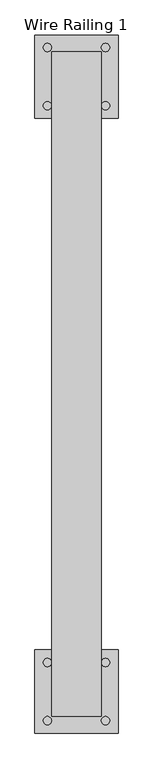
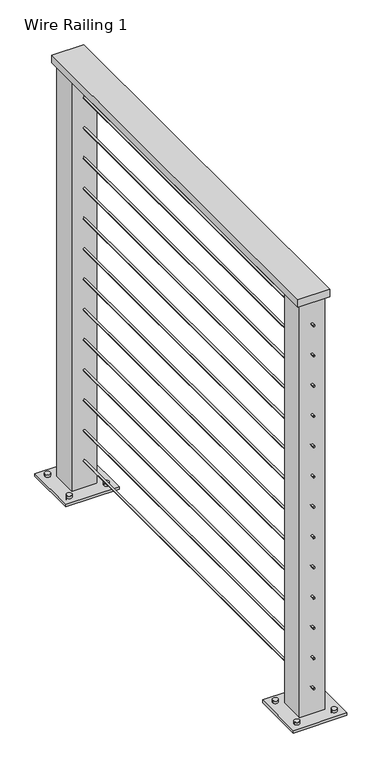
"""IFC4 building model written with IfcOpenShell, lengths in millimetres: railing geometry, Wire Railing 1."""

from ifc_helpers import new_model, si_unit, point, frame, frame_2d, origin, place, context, project, spatial, polyline, circle_curve, trimmed, segment, composite_curve, outline, extrude, source, transform, mapped, element, save


def wire_railing_1_44f17264(model_context):
    return source(origin(), model_context, "Body", "SweptSolid", [
        extrude(outline(polyline([(26672.156657, 26746.8531612), (26595.956657, 26746.8531612), (26595.956657, 27762.8531612), (26672.156657, 27762.8531612), (26672.156657, 26746.8531612)])), frame((0.0, 0.0, 270249.65), z_axis=(0.0, 0.0, 1.0), x_axis=(1.0, 0.0, 0.0)), (0.0, 0.0, 1.0), 19.05),
        extrude(outline(composite_curve([segment(trimmed(circle_curve(frame_2d((270190.11875, 26634.056657)), 2.38125), [point((270190.11875, 26631.675407))], [point((270190.11875, 26636.437907))], False, "CARTESIAN"), True, "CONTINUOUS"), segment(trimmed(circle_curve(frame_2d((270190.11875, 26634.056657)), 2.38125), [point((270190.11875, 26636.437907))], [point((270190.11875, 26631.675407))], False, "CARTESIAN"), True, "CONTINUOUS")], self_intersect=False)), frame((0.0, 26746.8531612, 0.0), z_axis=(0.0, 1.0, 0.0), x_axis=(0.0, 0.0, 1.0)), (0.0, 0.0, 1.0), 1016.0),
        extrude(outline(composite_curve([segment(trimmed(circle_curve(frame_2d((270113.91875, 26634.056657)), 2.38125), [point((270113.91875, 26631.675407))], [point((270113.91875, 26636.437907))], False, "CARTESIAN"), True, "CONTINUOUS"), segment(trimmed(circle_curve(frame_2d((270113.91875, 26634.056657)), 2.38125), [point((270113.91875, 26636.437907))], [point((270113.91875, 26631.675407))], False, "CARTESIAN"), True, "CONTINUOUS")], self_intersect=False)), frame((0.0, 26746.8531612, 0.0), z_axis=(0.0, 1.0, 0.0), x_axis=(0.0, 0.0, 1.0)), (0.0, 0.0, 1.0), 1016.0),
        extrude(outline(composite_curve([segment(trimmed(circle_curve(frame_2d((270037.71875, 26634.056657)), 2.38125), [point((270037.71875, 26631.675407))], [point((270037.71875, 26636.437907))], False, "CARTESIAN"), True, "CONTINUOUS"), segment(trimmed(circle_curve(frame_2d((270037.71875, 26634.056657)), 2.38125), [point((270037.71875, 26636.437907))], [point((270037.71875, 26631.675407))], False, "CARTESIAN"), True, "CONTINUOUS")], self_intersect=False)), frame((0.0, 26746.8531612, 0.0), z_axis=(0.0, 1.0, 0.0), x_axis=(0.0, 0.0, 1.0)), (0.0, 0.0, 1.0), 1016.0),
        extrude(outline(composite_curve([segment(trimmed(circle_curve(frame_2d((269961.51875, 26634.056657)), 2.38125), [point((269961.51875, 26631.675407))], [point((269961.51875, 26636.437907))], False, "CARTESIAN"), True, "CONTINUOUS"), segment(trimmed(circle_curve(frame_2d((269961.51875, 26634.056657)), 2.38125), [point((269961.51875, 26636.437907))], [point((269961.51875, 26631.675407))], False, "CARTESIAN"), True, "CONTINUOUS")], self_intersect=False)), frame((0.0, 26746.8531612, 0.0), z_axis=(0.0, 1.0, 0.0), x_axis=(0.0, 0.0, 1.0)), (0.0, 0.0, 1.0), 1016.0),
        extrude(outline(composite_curve([segment(trimmed(circle_curve(frame_2d((269885.31875, 26634.056657)), 2.38125), [point((269885.31875, 26631.675407))], [point((269885.31875, 26636.437907))], False, "CARTESIAN"), True, "CONTINUOUS"), segment(trimmed(circle_curve(frame_2d((269885.31875, 26634.056657)), 2.38125), [point((269885.31875, 26636.437907))], [point((269885.31875, 26631.675407))], False, "CARTESIAN"), True, "CONTINUOUS")], self_intersect=False)), frame((0.0, 26746.8531612, 0.0), z_axis=(0.0, 1.0, 0.0), x_axis=(0.0, 0.0, 1.0)), (0.0, 0.0, 1.0), 1016.0),
        extrude(outline(composite_curve([segment(trimmed(circle_curve(frame_2d((269809.11875, 26634.056657)), 2.38125), [point((269809.11875, 26631.675407))], [point((269809.11875, 26636.437907))], False, "CARTESIAN"), True, "CONTINUOUS"), segment(trimmed(circle_curve(frame_2d((269809.11875, 26634.056657)), 2.38125), [point((269809.11875, 26636.437907))], [point((269809.11875, 26631.675407))], False, "CARTESIAN"), True, "CONTINUOUS")], self_intersect=False)), frame((0.0, 26746.8531612, 0.0), z_axis=(0.0, 1.0, 0.0), x_axis=(0.0, 0.0, 1.0)), (0.0, 0.0, 1.0), 1016.0),
        extrude(outline(composite_curve([segment(trimmed(circle_curve(frame_2d((269732.91875, 26634.056657)), 2.38125), [point((269732.91875, 26631.675407))], [point((269732.91875, 26636.437907))], False, "CARTESIAN"), True, "CONTINUOUS"), segment(trimmed(circle_curve(frame_2d((269732.91875, 26634.056657)), 2.38125), [point((269732.91875, 26636.437907))], [point((269732.91875, 26631.675407))], False, "CARTESIAN"), True, "CONTINUOUS")], self_intersect=False)), frame((0.0, 26746.8531612, 0.0), z_axis=(0.0, 1.0, 0.0), x_axis=(0.0, 0.0, 1.0)), (0.0, 0.0, 1.0), 1016.0),
        extrude(outline(composite_curve([segment(trimmed(circle_curve(frame_2d((269656.71875, 26634.056657)), 2.38125), [point((269656.71875, 26631.675407))], [point((269656.71875, 26636.437907))], False, "CARTESIAN"), True, "CONTINUOUS"), segment(trimmed(circle_curve(frame_2d((269656.71875, 26634.056657)), 2.38125), [point((269656.71875, 26636.437907))], [point((269656.71875, 26631.675407))], False, "CARTESIAN"), True, "CONTINUOUS")], self_intersect=False)), frame((0.0, 26746.8531612, 0.0), z_axis=(0.0, 1.0, 0.0), x_axis=(0.0, 0.0, 1.0)), (0.0, 0.0, 1.0), 1016.0),
        extrude(outline(composite_curve([segment(trimmed(circle_curve(frame_2d((269580.51875, 26634.056657)), 2.38125), [point((269580.51875, 26631.675407))], [point((269580.51875, 26636.437907))], False, "CARTESIAN"), True, "CONTINUOUS"), segment(trimmed(circle_curve(frame_2d((269580.51875, 26634.056657)), 2.38125), [point((269580.51875, 26636.437907))], [point((269580.51875, 26631.675407))], False, "CARTESIAN"), True, "CONTINUOUS")], self_intersect=False)), frame((0.0, 26746.8531612, 0.0), z_axis=(0.0, 1.0, 0.0), x_axis=(0.0, 0.0, 1.0)), (0.0, 0.0, 1.0), 1016.0),
        extrude(outline(composite_curve([segment(trimmed(circle_curve(frame_2d((269504.31875, 26634.056657)), 2.38125), [point((269504.31875, 26631.675407))], [point((269504.31875, 26636.437907))], False, "CARTESIAN"), True, "CONTINUOUS"), segment(trimmed(circle_curve(frame_2d((269504.31875, 26634.056657)), 2.38125), [point((269504.31875, 26636.437907))], [point((269504.31875, 26631.675407))], False, "CARTESIAN"), True, "CONTINUOUS")], self_intersect=False)), frame((0.0, 26746.8531612, 0.0), z_axis=(0.0, 1.0, 0.0), x_axis=(0.0, 0.0, 1.0)), (0.0, 0.0, 1.0), 1016.0),
        extrude(outline(composite_curve([segment(trimmed(circle_curve(frame_2d((269428.11875, 26634.056657)), 2.38125), [point((269428.11875, 26631.675407))], [point((269428.11875, 26636.437907))], False, "CARTESIAN"), True, "CONTINUOUS"), segment(trimmed(circle_curve(frame_2d((269428.11875, 26634.056657)), 2.38125), [point((269428.11875, 26636.437907))], [point((269428.11875, 26631.675407))], False, "CARTESIAN"), True, "CONTINUOUS")], self_intersect=False)), frame((0.0, 26746.8531612, 0.0), z_axis=(0.0, 1.0, 0.0), x_axis=(0.0, 0.0, 1.0)), (0.0, 0.0, 1.0), 1016.0),
        extrude(outline(composite_curve([segment(trimmed(circle_curve(frame_2d((269351.91875, 26634.056657)), 2.38125), [point((269351.91875, 26631.675407))], [point((269351.91875, 26636.437907))], False, "CARTESIAN"), True, "CONTINUOUS"), segment(trimmed(circle_curve(frame_2d((269351.91875, 26634.056657)), 2.38125), [point((269351.91875, 26636.437907))], [point((269351.91875, 26631.675407))], False, "CARTESIAN"), True, "CONTINUOUS")], self_intersect=False)), frame((0.0, 26746.8531612, 0.0), z_axis=(0.0, 1.0, 0.0), x_axis=(0.0, 0.0, 1.0)), (0.0, 0.0, 1.0), 1016.0),
        extrude(outline(composite_curve([segment(trimmed(circle_curve(frame_2d((269275.71875, 26634.056657)), 2.38125), [point((269275.71875, 26631.675407))], [point((269275.71875, 26636.437907))], False, "CARTESIAN"), True, "CONTINUOUS"), segment(trimmed(circle_curve(frame_2d((269275.71875, 26634.056657)), 2.38125), [point((269275.71875, 26636.437907))], [point((269275.71875, 26631.675407))], False, "CARTESIAN"), True, "CONTINUOUS")], self_intersect=False)), frame((0.0, 26746.8531612, 0.0), z_axis=(0.0, 1.0, 0.0), x_axis=(0.0, 0.0, 1.0)), (0.0, 0.0, 1.0), 1016.0),
        extrude(outline(composite_curve([segment(trimmed(circle_curve(frame_2d((26678.506657, 27680.3031612)), 6.35), [point((26684.856657, 27680.3031612))], [point((26672.156657, 27680.3031612))], False, "CARTESIAN"), True, "CONTINUOUS"), segment(trimmed(circle_curve(frame_2d((26678.506657, 27680.3031612)), 6.35), [point((26672.156657, 27680.3031612))], [point((26684.856657, 27680.3031612))], False, "CARTESIAN"), True, "CONTINUOUS")], self_intersect=False)), frame((0.0, 0.0, 269201.9), z_axis=(0.0, 0.0, 1.0), x_axis=(1.0, 0.0, 0.0)), (0.0, 0.0, 1.0), 12.7),
        extrude(outline(composite_curve([segment(trimmed(circle_curve(frame_2d((26589.606657, 27680.3031612)), 6.35), [point((26595.956657, 27680.3031612))], [point((26583.256657, 27680.3031612))], False, "CARTESIAN"), True, "CONTINUOUS"), segment(trimmed(circle_curve(frame_2d((26589.606657, 27680.3031612)), 6.35), [point((26583.256657, 27680.3031612))], [point((26595.956657, 27680.3031612))], False, "CARTESIAN"), True, "CONTINUOUS")], self_intersect=False)), frame((0.0, 0.0, 269201.9), z_axis=(0.0, 0.0, 1.0), x_axis=(1.0, 0.0, 0.0)), (0.0, 0.0, 1.0), 12.7),
        extrude(outline(composite_curve([segment(trimmed(circle_curve(frame_2d((26678.506657, 27769.2031612)), 6.35), [point((26684.856657, 27769.2031612))], [point((26672.156657, 27769.2031612))], False, "CARTESIAN"), True, "CONTINUOUS"), segment(trimmed(circle_curve(frame_2d((26678.506657, 27769.2031612)), 6.35), [point((26672.156657, 27769.2031612))], [point((26684.856657, 27769.2031612))], False, "CARTESIAN"), True, "CONTINUOUS")], self_intersect=False)), frame((0.0, 0.0, 269201.9), z_axis=(0.0, 0.0, 1.0), x_axis=(1.0, 0.0, 0.0)), (0.0, 0.0, 1.0), 12.7),
        extrude(outline(composite_curve([segment(trimmed(circle_curve(frame_2d((26589.606657, 27769.2031612)), 6.35), [point((26595.956657, 27769.2031612))], [point((26583.256657, 27769.2031612))], False, "CARTESIAN"), True, "CONTINUOUS"), segment(trimmed(circle_curve(frame_2d((26589.606657, 27769.2031612)), 6.35), [point((26583.256657, 27769.2031612))], [point((26595.956657, 27769.2031612))], False, "CARTESIAN"), True, "CONTINUOUS")], self_intersect=False)), frame((0.0, 0.0, 269201.9), z_axis=(0.0, 0.0, 1.0), x_axis=(1.0, 0.0, 0.0)), (0.0, 0.0, 1.0), 12.7),
        extrude(outline(polyline([(26570.556657, 27661.2531612), (26570.556657, 27788.2531612), (26697.556657, 27788.2531612), (26697.556657, 27661.2531612), (26570.556657, 27661.2531612)])), frame((0.0, 0.0, 269201.9), z_axis=(0.0, 0.0, 1.0), x_axis=(1.0, 0.0, 0.0)), (0.0, 0.0, 1.0), 6.35),
        extrude(outline(polyline([(26603.894157, 27694.5906612), (26603.894157, 27754.9156612), (26664.219157, 27754.9156612), (26664.219157, 27694.5906612), (26603.894157, 27694.5906612)]), holes=[polyline([(26610.244157, 27700.9406612), (26657.869157, 27700.9406612), (26657.869157, 27748.5656612), (26610.244157, 27748.5656612), (26610.244157, 27700.9406612)])]), frame((0.0, 0.0, 269201.9), z_axis=(0.0, 0.0, 1.0), x_axis=(1.0, 0.0, 0.0)), (0.0, 0.0, 1.0), 1047.75),
        extrude(outline(composite_curve([segment(trimmed(circle_curve(frame_2d((26678.506657, 26740.5031612)), 6.35), [point((26684.856657, 26740.5031612))], [point((26672.156657, 26740.5031612))], False, "CARTESIAN"), True, "CONTINUOUS"), segment(trimmed(circle_curve(frame_2d((26678.506657, 26740.5031612)), 6.35), [point((26672.156657, 26740.5031612))], [point((26684.856657, 26740.5031612))], False, "CARTESIAN"), True, "CONTINUOUS")], self_intersect=False)), frame((0.0, 0.0, 269201.9), z_axis=(0.0, 0.0, 1.0), x_axis=(1.0, 0.0, 0.0)), (0.0, 0.0, 1.0), 12.7),
        extrude(outline(composite_curve([segment(trimmed(circle_curve(frame_2d((26589.606657, 26740.5031612)), 6.35), [point((26595.956657, 26740.5031612))], [point((26583.256657, 26740.5031612))], False, "CARTESIAN"), True, "CONTINUOUS"), segment(trimmed(circle_curve(frame_2d((26589.606657, 26740.5031612)), 6.35), [point((26583.256657, 26740.5031612))], [point((26595.956657, 26740.5031612))], False, "CARTESIAN"), True, "CONTINUOUS")], self_intersect=False)), frame((0.0, 0.0, 269201.9), z_axis=(0.0, 0.0, 1.0), x_axis=(1.0, 0.0, 0.0)), (0.0, 0.0, 1.0), 12.7),
        extrude(outline(composite_curve([segment(trimmed(circle_curve(frame_2d((26678.506657, 26829.4031612)), 6.35), [point((26684.856657, 26829.4031612))], [point((26672.156657, 26829.4031612))], False, "CARTESIAN"), True, "CONTINUOUS"), segment(trimmed(circle_curve(frame_2d((26678.506657, 26829.4031612)), 6.35), [point((26672.156657, 26829.4031612))], [point((26684.856657, 26829.4031612))], False, "CARTESIAN"), True, "CONTINUOUS")], self_intersect=False)), frame((0.0, 0.0, 269201.9), z_axis=(0.0, 0.0, 1.0), x_axis=(1.0, 0.0, 0.0)), (0.0, 0.0, 1.0), 12.7),
        extrude(outline(composite_curve([segment(trimmed(circle_curve(frame_2d((26589.606657, 26829.4031612)), 6.35), [point((26595.956657, 26829.4031612))], [point((26583.256657, 26829.4031612))], False, "CARTESIAN"), True, "CONTINUOUS"), segment(trimmed(circle_curve(frame_2d((26589.606657, 26829.4031612)), 6.35), [point((26583.256657, 26829.4031612))], [point((26595.956657, 26829.4031612))], False, "CARTESIAN"), True, "CONTINUOUS")], self_intersect=False)), frame((0.0, 0.0, 269201.9), z_axis=(0.0, 0.0, 1.0), x_axis=(1.0, 0.0, 0.0)), (0.0, 0.0, 1.0), 12.7),
        extrude(outline(polyline([(26570.556657, 26721.4531612), (26570.556657, 26848.4531612), (26697.556657, 26848.4531612), (26697.556657, 26721.4531612), (26570.556657, 26721.4531612)])), frame((0.0, 0.0, 269201.9), z_axis=(0.0, 0.0, 1.0), x_axis=(1.0, 0.0, 0.0)), (0.0, 0.0, 1.0), 6.35),
        extrude(outline(polyline([(26603.894157, 26754.7906612), (26603.894157, 26815.1156612), (26664.219157, 26815.1156612), (26664.219157, 26754.7906612), (26603.894157, 26754.7906612)]), holes=[polyline([(26610.244157, 26761.1406612), (26657.869157, 26761.1406612), (26657.869157, 26808.7656612), (26610.244157, 26808.7656612), (26610.244157, 26761.1406612)])]), frame((0.0, 0.0, 269201.9), z_axis=(0.0, 0.0, 1.0), x_axis=(1.0, 0.0, 0.0)), (0.0, 0.0, 1.0), 1047.75),
    ])


if __name__ == "__main__":
    model = new_model("IFC4")
    model_context = context("Model", 3, world=origin())
    ifc_project = project(units=[si_unit("LENGTHUNIT", "METRE", prefix="MILLI")], contexts=[model_context])
    site = spatial("IfcSite", under=ifc_project)
    building = spatial("IfcBuilding", under=site)
    placement = place(None, origin())
    wire_railing_1_shape = wire_railing_1_44f17264(model_context)
    element("IfcRailing", 1, ObjectType="Wire Railing 1", at=placement, inside=building, context=model_context, shape_type="MappedRepresentation", body=[
        mapped(wire_railing_1_shape, transform((0.0, 0.0, 0.0), x_axis=(1.0, 0.0, 0.0), y_axis=(0.0, 1.0, 0.0), z_axis=(0.0, 0.0, 1.0))),
    ])
    save(model, "model.ifc")

# Revit data of these elements
# Element 1 (IfcRailing, "Wire Railing 1")
#   Materials on its faces: "WIRE RAILING (3\" O.C.)", "2 1/2\" X 2 1/2\" ALUM. SQUARE POST (38\" O.C. MAX)", "ALUM. PLATE TOP RAIL"
# Materials
#   "WIRE RAILING (3\" O.C.)": class "Metal", colour RGB 244 244 244, transparency 0, Manufacturer = "Kawneer", URL = "http://www.kawneer.com/kawneer/north_america/en/home.asp", Cost = 0
#   "2 1/2\" X 2 1/2\" ALUM. SQUARE POST (38\" O.C. MAX)": class "Metal", colour RGB 244 244 244, transparency 0, Manufacturer = "Kawneer", URL = "http://www.kawneer.com/kawneer/north_america/en/home.asp", Cost = 0
#   "ALUM. PLATE TOP RAIL": class "Metal", colour RGB 244 244 244, transparency 0, Manufacturer = "Kawneer", URL = "http://www.kawneer.com/kawneer/north_america/en/home.asp", Cost = 0
